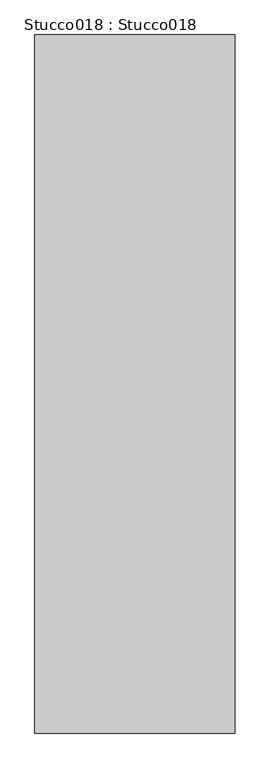
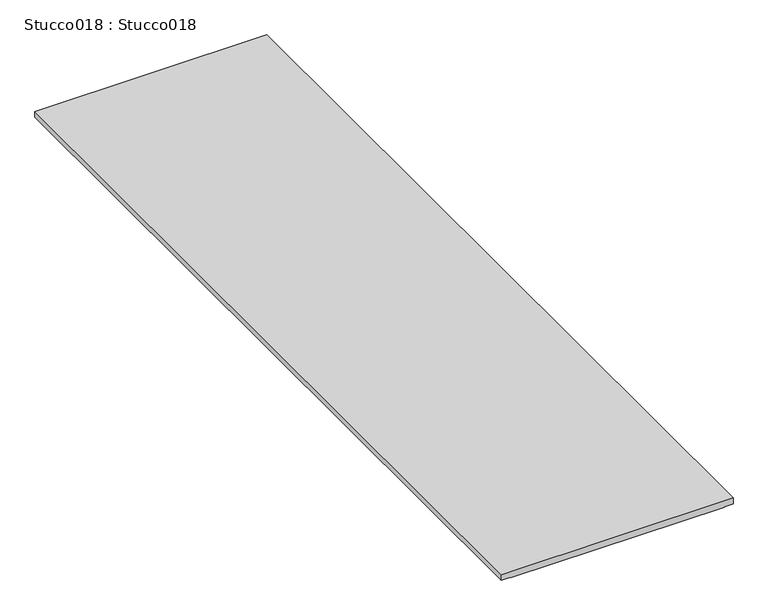
"""IFC4 building model written with IfcOpenShell, lengths in millimetres: proxy geometry, Stucco018 : Stucco018."""

import ifcopenshell
import ifcopenshell.guid

model = None  # the IFC model being written
_history = None  # IfcOwnerHistory: only IFC2X3 demands one
_inside = {}  # id of a spatial element -> (the spatial element, [elements in it])
_under = {}  # id of a project, library or spatial element -> (it, [spatial elements below it])
_declared = {}  # id of a project -> (the project, [libraries it declares])
_typed = {}  # id of a type object -> (the type object, [elements of that type])
_made_of = {}  # id of a material, layer set ... -> (it, [elements and type objects made of it])


def new_model(schema):
    """Start an empty IFC model of exactly this schema.

    Asked for "IFC4X3", IfcOpenShell would pick the latest addendum, in which some entities
    have other attributes; the version numbers below select the first issue.
    IFC2X3 requires an IfcOwnerHistory on every rooted entity: one is made here for all.
    """
    global model, _history
    if schema == "IFC4X3":
        model = ifcopenshell.file(schema_version=(4, 3, 0, 0))
    else:
        model = ifcopenshell.file(schema=schema)
    _inside.clear()
    _under.clear()
    _declared.clear()
    _typed.clear()
    _made_of.clear()
    _history = None
    if model.schema == "IFC2X3":
        org = make("IfcOrganization", Name="unknown")
        user = make(
            "IfcPersonAndOrganization",
            ThePerson=make("IfcPerson", FamilyName="unknown"),
            TheOrganization=org,
        )
        app = make(
            "IfcApplication",
            ApplicationDeveloper=org,
            Version="unknown",
            ApplicationFullName="unknown",
            ApplicationIdentifier="unknown",
        )
        _history = make(
            "IfcOwnerHistory",
            OwningUser=user,
            OwningApplication=app,
            ChangeAction="ADDED",
            CreationDate=0,
        )
    return model


def make(cls, **values):
    """One entity of the class cls with the attributes given. An attribute that is None is left unset."""
    return model.create_entity(
        cls, **{name: value for name, value in values.items() if value is not None}
    )


def rooted(cls, **values):
    """An entity with a GlobalId (a new one), such as an element, a storey or a relation."""
    return make(cls, GlobalId=ifcopenshell.guid.new(), OwnerHistory=_history, **values)


def si_unit(unit_type, name, prefix=None):
    """IfcSIUnit, for example si_unit("LENGTHUNIT", "METRE", prefix="MILLI")."""
    return make("IfcSIUnit", UnitType=unit_type, Prefix=prefix, Name=name)


def assignment(units):
    """IfcUnitAssignment: the units of a project."""
    return None if units is None else make("IfcUnitAssignment", Units=units)


def point(xyz):
    """IfcCartesianPoint."""
    return None if xyz is None else make("IfcCartesianPoint", Coordinates=xyz)


def direction(xyz):
    """IfcDirection."""
    return None if xyz is None else make("IfcDirection", DirectionRatios=xyz)


def frame(location, z_axis=None, x_axis=None):
    """IfcAxis2Placement3D, a coordinate frame: its origin and axes. An axis left out is left unset."""
    return make(
        "IfcAxis2Placement3D",
        Location=point(location),
        Axis=direction(z_axis),
        RefDirection=direction(x_axis),
    )


def origin():
    """The frame at (0, 0, 0) with its axes left unset."""
    return frame((0.0, 0.0, 0.0))


def place(relative_to, where):
    """IfcLocalPlacement: puts the frame where relative to a parent placement (None: the world)."""
    return make(
        "IfcLocalPlacement", PlacementRelTo=relative_to, RelativePlacement=where
    )


def context(
    kind, dimensions, precision=None, world=None, true_north=None, identifier=None
):
    """IfcGeometricRepresentationContext, for example the 3D "Model" context."""
    return make(
        "IfcGeometricRepresentationContext",
        ContextIdentifier=identifier,
        ContextType=kind,
        CoordinateSpaceDimension=dimensions,
        Precision=precision,
        WorldCoordinateSystem=world,
        TrueNorth=true_north,
    )


def project(units=None, contexts=None):
    """IfcProject with its units and contexts."""
    return rooted(
        "IfcProject",
        Name="project",
        RepresentationContexts=contexts,
        UnitsInContext=assignment(units),
    )


def spatial(cls, under=None, at=None, **own):
    """A site, building, storey or space (cls), placed at a placement, below another one or the project."""
    s = rooted(cls, ObjectPlacement=at, **own)
    if under is not None:
        _under.setdefault(under.id(), (under, []))[1].append(s)
    return s


def polyline(points):
    """IfcPolyline through the points."""
    return make("IfcPolyline", Points=[point(p) for p in points])


def outline(outer, holes=None, kind="AREA"):
    """IfcArbitraryClosedProfileDef: a profile drawn as a closed curve; with holes, ...WithVoids."""
    if holes is None:
        return make("IfcArbitraryClosedProfileDef", ProfileType=kind, OuterCurve=outer)
    return make(
        "IfcArbitraryProfileDefWithVoids",
        ProfileType=kind,
        OuterCurve=outer,
        InnerCurves=holes,
    )


def extrude(swept, where, along, depth):
    """IfcExtrudedAreaSolid: the profile swept, set in the frame where, extruded along a direction by depth."""
    return make(
        "IfcExtrudedAreaSolid",
        SweptArea=swept,
        Position=where,
        ExtrudedDirection=direction(along),
        Depth=depth,
    )


def shape(context_of_items, identifier, shape_type, items):
    """IfcShapeRepresentation: the items that make up one representation, for example the "Body"."""
    return make(
        "IfcShapeRepresentation",
        ContextOfItems=context_of_items,
        RepresentationIdentifier=identifier,
        RepresentationType=shape_type,
        Items=items,
    )


def source(mapping_origin, context_of_items, identifier, shape_type, items):
    """IfcRepresentationMap: a shape defined once, which mapped items show again and again."""
    return make(
        "IfcRepresentationMap",
        MappingOrigin=mapping_origin,
        MappedRepresentation=shape(context_of_items, identifier, shape_type, items),
    )


def transform(
    local_origin,
    x_axis=None,
    y_axis=None,
    z_axis=None,
    scale=None,
    scale2=None,
    scale3=None,
    uniform=True,
):
    """IfcCartesianTransformationOperator3D, or its non-uniform kind. x_axis, y_axis, z_axis: its Axis1, 2, 3."""
    if uniform:
        return make(
            "IfcCartesianTransformationOperator3D",
            Axis1=direction(x_axis),
            Axis2=direction(y_axis),
            LocalOrigin=point(local_origin),
            Scale=scale,
            Axis3=direction(z_axis),
        )
    return make(
        "IfcCartesianTransformationOperator3DnonUniform",
        Axis1=direction(x_axis),
        Axis2=direction(y_axis),
        LocalOrigin=point(local_origin),
        Scale=scale,
        Axis3=direction(z_axis),
        Scale2=scale2,
        Scale3=scale3,
    )


def mapped(mapping_source, mapping_target):
    """IfcMappedItem: shows the shape of a source again, moved by a transform."""
    return make(
        "IfcMappedItem", MappingSource=mapping_source, MappingTarget=mapping_target
    )


def made_of(thing, what):
    """Note that an element or type object is made of a material, layer set ...; save() writes the relation."""
    if what is not None:
        _made_of.setdefault(what.id(), (what, []))[1].append(thing)
    return thing


def element(
    cls,
    number,
    at=None,
    inside=None,
    cuts=None,
    type_object=None,
    material=None,
    context=None,
    identifier="Body",
    shape_type=None,
    held_by="IfcProductDefinitionShape",
    body=None,
    shapes=None,
    **own,
):
    """One element of the class cls, such as IfcWall. Its Tag is "e" and its number.

    at: its placement. inside: the storey or other place that contains it. cuts: it is an
    opening in that element (IfcRelVoidsElement). A single representation is given by context,
    identifier, shape_type and body (its items); several are given by shapes. held_by: the class
    of the entity that holds the representations. save() writes the other relations.
    """
    e = rooted(cls, Tag="e%d" % number, ObjectPlacement=at, **own)
    if body is not None:
        shapes = [shape(context, identifier, shape_type, body)]
    if shapes is not None:
        e.Representation = make(held_by, Representations=shapes)
    if inside is not None:
        _inside.setdefault(inside.id(), (inside, []))[1].append(e)
    if cuts is not None:
        rooted(
            "IfcRelVoidsElement", RelatingBuildingElement=cuts, RelatedOpeningElement=e
        )
    if type_object is not None:
        _typed.setdefault(type_object.id(), (type_object, []))[1].append(e)
    return made_of(e, material)


def aggregate(whole, parts):
    """IfcRelAggregates: a whole, such as a stair, and the parts it consists of."""
    return rooted("IfcRelAggregates", RelatingObject=whole, RelatedObjects=parts)


def save(model, path):
    """Write the relations noted so far, then the file.

    IfcRelAggregates (storeys below a building ...), IfcRelContainedInSpatialStructure (elements
    in a storey), IfcRelDefinesByType, IfcRelAssociatesMaterial and IfcRelDeclares: one each for
    every whole, place, type object, material and project.
    """
    for whole, parts in _under.values():
        aggregate(whole, parts)
    for where, things in _inside.values():
        rooted(
            "IfcRelContainedInSpatialStructure",
            RelatedElements=things,
            RelatingStructure=where,
        )
    for kind, things in _typed.values():
        rooted("IfcRelDefinesByType", RelatedObjects=things, RelatingType=kind)
    for what, things in _made_of.values():
        rooted("IfcRelAssociatesMaterial", RelatedObjects=things, RelatingMaterial=what)
    for by, libraries in _declared.values():
        rooted("IfcRelDeclares", RelatingContext=by, RelatedDefinitions=libraries)
    model.write(path)


def stucco018_stucco018_7d097d3a(model_context):
    return source(origin(), model_context, "Body", "SweptSolid", [
        extrude(outline(polyline([(39545.1675708, -9856.7873925), (39543.8875708, -9856.7873925), (39543.8875708, -9328.1369192), (39545.1675708, -9328.1369192), (39545.1675708, -9305.7037353), (39560.2460083, -9305.7037353), (39560.2460083, -9879.2205764), (39545.1675708, -9879.2205764), (39545.1675708, -9856.7873925)])), frame((0.0, 7982.1531721, 0.0), z_axis=(0.0, 1.0, 0.0), x_axis=(0.0, 0.0, 1.0)), (0.0, 0.0, 1.0), 2000.0),
    ])


if __name__ == "__main__":
    model = new_model("IFC4")
    model_context = context("Model", 3, world=origin())
    ifc_project = project(units=[si_unit("LENGTHUNIT", "METRE", prefix="MILLI")], contexts=[model_context])
    site = spatial("IfcSite", under=ifc_project)
    building = spatial("IfcBuilding", under=site)
    placement = place(None, origin())
    stucco018_stucco018_shape = stucco018_stucco018_7d097d3a(model_context)
    element("IfcBuildingElementProxy", 1, Name="Stucco018 : Stucco018", ObjectType="Stucco018 : Stucco018", at=placement, inside=building, context=model_context, shape_type="MappedRepresentation", body=[
        mapped(stucco018_stucco018_shape, transform((0.0, 0.0, 0.0), x_axis=(1.0, 0.0, 0.0), y_axis=(0.0, 1.0, 0.0), z_axis=(0.0, 0.0, 1.0))),
    ])
    save(model, "model.ifc")

# Revit data of these elements
# Type "Stucco018 : Stucco018"
#   NameOverride = "Stucco018"
# Element 1 (IfcBuildingElementProxy, "Stucco018 : Stucco018")
#   Materials on its faces: "7/8\" SMOOTH TROWEL EXTERIOR STUCCO"
# Materials
#   "7/8\" SMOOTH TROWEL EXTERIOR STUCCO": class "Unassigned", colour RGB 255 255 255, transparency 0, Cost = 0
